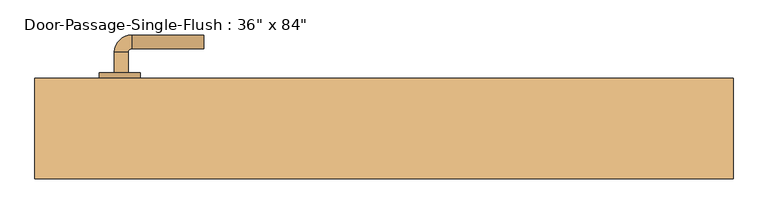
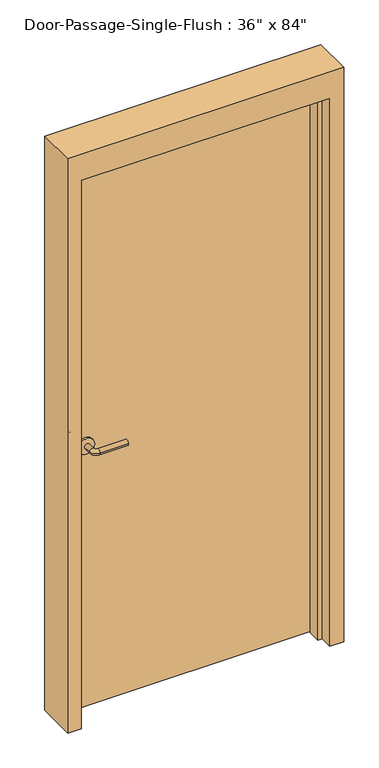
"""IFC4 building model written with IfcOpenShell, lengths in millimetres: door geometry."""

from ifc_helpers import new_model, si_unit, point, frame, frame_2d, origin, origin_with_axes, place, context, project, spatial, polyline, circle_curve, ellipse_curve, trimmed, segment, composite_curve, outline, extrude, faceted_brep, source, transform, mapped, element, save
from ifc_brep_helpers import plane_surface, cylinder_surface, revolved_surface, advanced_brep


def door_e56c0533(model_context):
    return source(origin(), model_context, "Body", "SolidModel", [
        advanced_brep(
        [(-392.190625, 76.1375, 1016.0), (-372.190625, 76.1375, 1016.0), (-372.190625, 46.1375, 1016.0), (-392.190625, 46.1375, 1016.0), (-367.190625, 41.1375, 1016.0), (-367.190625, 21.1375, 1016.0), (-262.190625, 21.1375, 1016.0), (-262.190625, 41.1375, 1016.0)],
        [
            (0, 1, circle_curve(frame((-382.190625, 76.1375, 1016.0), z_axis=(0.0, 1.0, 0.0), x_axis=(1.0, 0.0, 0.0)), 10.0)),
            (1, 0, circle_curve(frame((-382.190625, 76.1375, 1016.0), z_axis=(0.0, 1.0, 0.0), x_axis=(1.0, 0.0, 0.0)), 10.0)),
            (1, 2),
            (2, 3, circle_curve(frame((-382.190625, 46.1375, 1016.0), z_axis=(0.0, 1.0, 0.0), x_axis=(1.0, 0.0, 0.0)), 10.0)),
            (3, 0),
            (3, 2, circle_curve(frame((-382.190625, 46.1375, 1016.0), z_axis=(0.0, 1.0, 0.0), x_axis=(1.0, 0.0, 0.0)), 10.0)),
            (4, 5, circle_curve(frame((-367.190625, 31.1375, 1016.0), z_axis=(-1.0, 0.0, 0.0), x_axis=(0.0, 1.0, 0.0)), 10.0)),
            (5, 3, circle_curve(frame((-367.190625, 46.1375, 1016.0), z_axis=(0.0, 0.0, -1.0), x_axis=(-1.0, 0.0, 0.0)), 25.0)),
            (2, 4, circle_curve(frame((-367.190625, 46.1375, 1016.0), z_axis=(0.0, 0.0, 1.0), x_axis=(-1.0, 0.0, 0.0)), 5.0)),
            (5, 4, circle_curve(frame((-367.190625, 31.1375, 1016.0), z_axis=(-1.0, 0.0, 0.0), x_axis=(0.0, 1.0, 0.0)), 10.0)),
            (6, 7, circle_curve(frame((-262.190625, 31.1375, 1016.0), z_axis=(1.0, 0.0, 0.0), x_axis=(0.0, 1.0, 0.0)), 10.0)),
            (7, 6, circle_curve(frame((-262.190625, 31.1375, 1016.0), z_axis=(1.0, 0.0, 0.0), x_axis=(0.0, 1.0, 0.0)), 10.0)),
            (4, 7),
            (6, 5),
        ],
        [
            plane_surface(frame((-382.190625, 76.1375, 1016.0), z_axis=(0.0, 1.0, 0.0), x_axis=(0.0, 0.0, 1.0))),
            cylinder_surface(frame((-382.190625, 76.1375, 1016.0), z_axis=(0.0, 1.0, 0.0), x_axis=(1.0, 0.0, 0.0)), 10.0),
            revolved_surface(trimmed(ellipse_curve(frame((-382.190625, 46.1375, 1016.0), z_axis=(0.0, -1.0, 0.0), x_axis=(1.0, 0.0, 0.0)), 10.0, 10.0), [point((-392.190625, 46.1375, 1016.0))], [point((-372.190625, 46.1375, 1016.0))], True, "CARTESIAN"), (-367.190625, 46.1375, 1016.0), (0.0, 0.0, -1.0)),
            revolved_surface(trimmed(ellipse_curve(frame((-382.190625, 46.1375, 1016.0), z_axis=(0.0, -1.0, 0.0), x_axis=(1.0, 0.0, 0.0)), 10.0, 10.0), [point((-372.190625, 46.1375, 1016.0))], [point((-392.190625, 46.1375, 1016.0))], True, "CARTESIAN"), (-367.190625, 46.1375, 1016.0), (0.0, 0.0, -1.0)),
            plane_surface(frame((-262.190625, 31.1375, 1016.0), z_axis=(1.0, 0.0, 0.0), x_axis=(0.0, 0.0, 1.0))),
            cylinder_surface(frame((-367.190625, 31.1375, 1016.0), z_axis=(-1.0, 0.0, 0.0), x_axis=(0.0, 1.0, 0.0)), 10.0),
        ],
        [
            (0, [[1, 2]]),
            (1, [[3, 4, 5, -2]]),
            (1, [[-5, 6, -3, -1]]),
            (2, [[7, 8, -4, 9]]),
            (3, [[10, -9, -6, -8]]),
            (4, [[11, 12]]),
            (5, [[13, -11, 14, -7]]),
            (5, [[-14, -12, -13, -10]]),
        ],
    ),
        extrude(outline(composite_curve([segment(trimmed(circle_curve(frame_2d((1016.0, -384.690625)), 30.0), [point((1016.0, -414.690625))], [point((1016.0, -354.690625))], False, "CARTESIAN"), True, "CONTINUOUS"), segment(trimmed(circle_curve(frame_2d((1016.0, -384.690625)), 30.0), [point((1016.0, -354.690625))], [point((1016.0, -414.690625))], False, "CARTESIAN"), True, "CONTINUOUS")], self_intersect=False)), frame((0.0, 76.1375, 0.0), z_axis=(0.0, 1.0, 0.0), x_axis=(0.0, 0.0, 1.0)), (0.0, 0.0, 1.0), 8.0),
        advanced_brep(
        [(-392.190625, 136.5875, 1016.0), (-372.190625, 136.5875, 1016.0), (-392.190625, 166.5875, 1016.0), (-372.190625, 166.5875, 1016.0), (-367.190625, 171.5875, 1016.0), (-367.190625, 191.5875, 1016.0), (-262.190625, 191.5875, 1016.0), (-262.190625, 171.5875, 1016.0)],
        [
            (0, 1, circle_curve(frame((-382.190625, 136.5875, 1016.0), z_axis=(0.0, -1.0, 0.0), x_axis=(1.0, 0.0, 0.0)), 10.0)),
            (1, 0, circle_curve(frame((-382.190625, 136.5875, 1016.0), z_axis=(0.0, -1.0, 0.0), x_axis=(1.0, 0.0, 0.0)), 10.0)),
            (0, 2),
            (2, 3, circle_curve(frame((-382.190625, 166.5875, 1016.0), z_axis=(0.0, -1.0, 0.0), x_axis=(1.0, 0.0, 0.0)), 10.0)),
            (3, 1),
            (3, 2, circle_curve(frame((-382.190625, 166.5875, 1016.0), z_axis=(0.0, -1.0, 0.0), x_axis=(1.0, 0.0, 0.0)), 10.0)),
            (4, 3, circle_curve(frame((-367.190625, 166.5875, 1016.0), z_axis=(0.0, 0.0, 1.0), x_axis=(-1.0, 0.0, 0.0)), 5.0)),
            (2, 5, circle_curve(frame((-367.190625, 166.5875, 1016.0), z_axis=(0.0, 0.0, -1.0), x_axis=(-1.0, 0.0, 0.0)), 25.0)),
            (5, 4, circle_curve(frame((-367.190625, 181.5875, 1016.0), z_axis=(-1.0, 0.0, 0.0), x_axis=(0.0, -1.0, 0.0)), 10.0)),
            (4, 5, circle_curve(frame((-367.190625, 181.5875, 1016.0), z_axis=(-1.0, 0.0, 0.0), x_axis=(0.0, -1.0, 0.0)), 10.0)),
            (6, 7, circle_curve(frame((-262.190625, 181.5875, 1016.0), z_axis=(1.0, 0.0, 0.0), x_axis=(0.0, -1.0, 0.0)), 10.0)),
            (7, 6, circle_curve(frame((-262.190625, 181.5875, 1016.0), z_axis=(1.0, 0.0, 0.0), x_axis=(0.0, -1.0, 0.0)), 10.0)),
            (5, 6),
            (7, 4),
        ],
        [
            plane_surface(frame((-382.190625, 136.5875, 1016.0), z_axis=(0.0, -1.0, 0.0), x_axis=(0.0, 0.0, 1.0))),
            cylinder_surface(frame((-382.190625, 136.5875, 1016.0), z_axis=(0.0, -1.0, 0.0), x_axis=(1.0, 0.0, 0.0)), 10.0),
            revolved_surface(trimmed(ellipse_curve(frame((-382.190625, 166.5875, 1016.0), z_axis=(0.0, -1.0, 0.0), x_axis=(1.0, 0.0, 0.0)), 10.0, 10.0), [point((-392.190625, 166.5875, 1016.0))], [point((-372.190625, 166.5875, 1016.0))], True, "CARTESIAN"), (-367.190625, 166.5875, 1016.0), (0.0, 0.0, -1.0)),
            revolved_surface(trimmed(ellipse_curve(frame((-382.190625, 166.5875, 1016.0), z_axis=(0.0, -1.0, 0.0), x_axis=(1.0, 0.0, 0.0)), 10.0, 10.0), [point((-372.190625, 166.5875, 1016.0))], [point((-392.190625, 166.5875, 1016.0))], True, "CARTESIAN"), (-367.190625, 166.5875, 1016.0), (0.0, 0.0, -1.0)),
            plane_surface(frame((-262.190625, 181.5875, 1016.0), z_axis=(1.0, 0.0, 0.0), x_axis=(0.0, 0.0, 1.0))),
            cylinder_surface(frame((-367.190625, 181.5875, 1016.0), z_axis=(-1.0, 0.0, 0.0), x_axis=(0.0, -1.0, 0.0)), 10.0),
        ],
        [
            (0, [[1, 2]]),
            (1, [[-1, 3, 4, 5]]),
            (1, [[-2, -5, 6, -3]]),
            (2, [[7, -4, 8, 9]]),
            (3, [[-8, -6, -7, 10]]),
            (4, [[11, 12]]),
            (5, [[-9, 13, -12, 14]]),
            (5, [[-10, -14, -11, -13]]),
        ],
    ),
        extrude(outline(composite_curve([segment(trimmed(circle_curve(frame_2d((1016.0, -384.690625)), 30.0), [point((1016.0, -414.690625))], [point((1016.0, -354.690625))], False, "CARTESIAN"), True, "CONTINUOUS"), segment(trimmed(circle_curve(frame_2d((1016.0, -384.690625)), 30.0), [point((1016.0, -354.690625))], [point((1016.0, -414.690625))], False, "CARTESIAN"), True, "CONTINUOUS")], self_intersect=False)), frame((0.0, 128.5875, 0.0), z_axis=(0.0, 1.0, 0.0), x_axis=(0.0, 0.0, 1.0)), (0.0, 0.0, 1.0), 8.0),
        faceted_brep([(457.2, 79.375, 0.0), (457.2, 128.5875, 0.0), (508.0, 128.5875, 0.0), (508.0, -17.4625, 0.0), (457.2, -17.4625, 0.0), (457.2, 31.75, 0.0), (441.325, 31.75, 0.0), (441.325, 79.375, 0.0), (457.2, 79.375, 2133.6), (457.2, 128.5875, 2133.6), (-457.2, 128.5875, 2133.6), (-457.2, 128.5875, 0.0), (-508.0, 128.5875, 0.0), (-508.0, 128.5875, 2235.2), (508.0, 128.5875, 2235.2), (508.0, -17.4625, 2235.2), (-508.0, -17.4625, 2235.2), (-508.0, -17.4625, 0.0), (-457.2, -17.4625, 0.0), (-457.2, -17.4625, 2133.6), (457.2, -17.4625, 2133.6), (457.2, 31.75, 2133.6), (-457.2, 31.75, 2133.6), (-457.2, 31.75, 0.0), (-441.325, 31.75, 0.0), (-441.325, 31.75, 2117.725), (441.325, 31.75, 2117.725), (441.325, 79.375, 2117.725), (-441.325, 79.375, 2117.725), (-441.325, 79.375, 0.0), (-457.2, 79.375, 0.0), (-457.2, 79.375, 2133.6)], [[[0, 1, 2, 3, 4, 5, 6, 7]], [[1, 0, 8, 9]], [[2, 1, 9, 10, 11, 12, 13, 14]], [[3, 2, 14, 15]], [[4, 3, 15, 16, 17, 18, 19, 20]], [[5, 4, 20, 21]], [[6, 5, 21, 22, 23, 24, 25, 26]], [[7, 6, 26, 27]], [[0, 7, 27, 28, 29, 30, 31, 8]], [[9, 8, 31, 10]], [[20, 19, 22, 21]], [[26, 25, 28, 27]], [[12, 11, 30, 29, 24, 23, 18, 17]], [[11, 10, 31, 30]], [[13, 12, 17, 16]], [[19, 18, 23, 22]], [[25, 24, 29, 28]], [[15, 14, 13, 16]]]),
        extrude(outline(polyline([(457.2, 84.1375), (-457.2, 84.1375), (-457.2, 128.5875), (457.2, 128.5875), (457.2, 84.1375)])), origin_with_axes(), (0.0, 0.0, 1.0), 2133.6),
    ])


if __name__ == "__main__":
    model = new_model("IFC4")
    model_context = context("Model", 3, world=origin())
    ifc_project = project(units=[si_unit("LENGTHUNIT", "METRE", prefix="MILLI")], contexts=[model_context])
    site = spatial("IfcSite", under=ifc_project)
    building = spatial("IfcBuilding", under=site)
    placement = place(None, origin())
    door_shape = door_e56c0533(model_context)
    element("IfcDoor", 1, ObjectType="Door-Passage-Single-Flush : 36\" x 84\"", at=placement, inside=building, context=model_context, shape_type="MappedRepresentation", body=[
        mapped(door_shape, transform((0.0, 0.0, 0.0), x_axis=(1.0, 0.0, 0.0), y_axis=(0.0, 1.0, 0.0), z_axis=(0.0, 0.0, 1.0))),
    ])
    save(model, "model.ifc")

# Revit data of these elements
# Type "Door-Passage-Single-Flush : 36\" x 84\""
#   Type Mark = "1"
#   Assembly Code = "B2030200"
#   Analytic Construction = "Wooden"
#   Thickness = 0' - 1 3/4"
#   Thermal Resistance (R) = 2.5876 (h·ft²·°F)/BTU
#   Swing Angle [instance default] = 90.00°
#   Strike Height = 3' - 4"
#   Rough Width [instance default] = 3' - 4"
#   Rough Height [instance default] = 7' - 4"
#   MF Opening Height [instance default] = 0' - 4"
#   MF Opening Width [instance default] = 0' - 4"
#   Inset Calculate [instance default] = 0' - 4"
#   Masonry Inset [instance default] = 0' - 1"
#   Height = 7' - 0"
#   Width = 3' - 0"
#   Heat Transfer Coefficient (U) = 0.3865 BTU/(h·ft²·°F)
#   Masonry Frame Depth = 0' - 5 3/4"
#   Define Thermal Properties by = 1
#   Masonry Frame [instance default] = yes
#   Function = 1
#   Dry Wall Frame [instance default] = no
#   Panel Material = Wood - Birch
#   Frame Material = Metal - Paint Finish - Grey
#   Door Handle Material = Aluminum
#   Visual Light Transmittance = 0
#   Solar Heat Gain Coefficient = 0
#   Wall Closure = (empty or 0)
# Element 1 (IfcDoor, "Door-Passage-Single-Flush : 36\" x 84\"")
#   Materials on its faces: "Aluminum", "Metal - Paint Finish - Grey", "Wood - Birch"
# Materials
#   "Wood - Birch": class "Wood", colour RGB 166 116 52, transparency 0, Cost = 0
#   "Metal - Paint Finish - Grey": class "Paint", colour RGB 104 104 104, transparency 0, Cost = 0
#   "Aluminum": class "Metal", colour RGB 247 247 247, transparency 0, Description = "Aluminum 6061", Cost = 0
